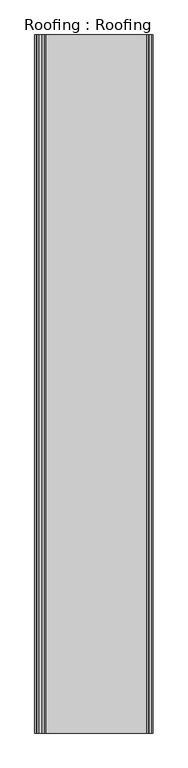
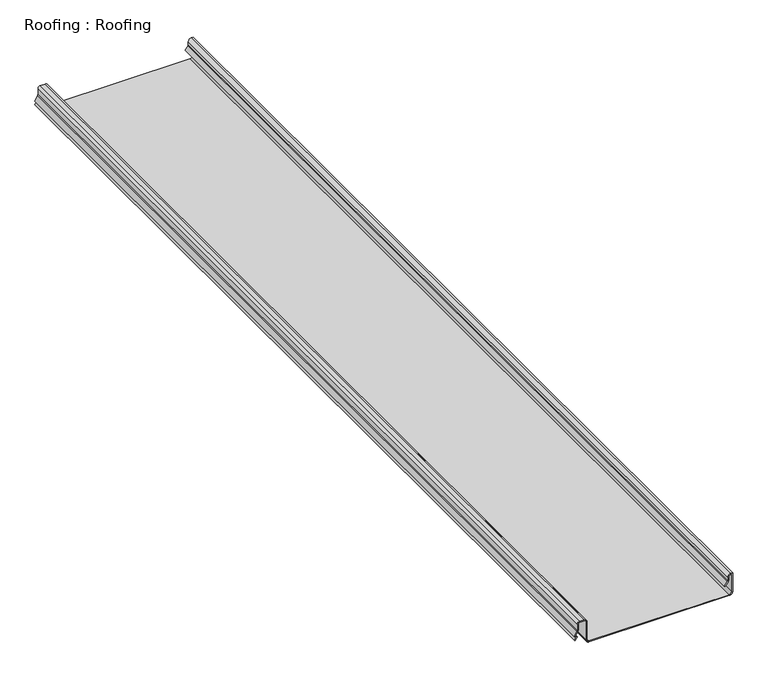
"""IFC4 building model written with IfcOpenShell, lengths in millimetres: proxy geometry, Roofing : Roofing."""

import ifcopenshell
import ifcopenshell.guid

model = None  # the IFC model being written
_history = None  # IfcOwnerHistory: only IFC2X3 demands one
_inside = {}  # id of a spatial element -> (the spatial element, [elements in it])
_under = {}  # id of a project, library or spatial element -> (it, [spatial elements below it])
_declared = {}  # id of a project -> (the project, [libraries it declares])
_typed = {}  # id of a type object -> (the type object, [elements of that type])
_made_of = {}  # id of a material, layer set ... -> (it, [elements and type objects made of it])


def new_model(schema):
    """Start an empty IFC model of exactly this schema.

    Asked for "IFC4X3", IfcOpenShell would pick the latest addendum, in which some entities
    have other attributes; the version numbers below select the first issue.
    IFC2X3 requires an IfcOwnerHistory on every rooted entity: one is made here for all.
    """
    global model, _history
    if schema == "IFC4X3":
        model = ifcopenshell.file(schema_version=(4, 3, 0, 0))
    else:
        model = ifcopenshell.file(schema=schema)
    _inside.clear()
    _under.clear()
    _declared.clear()
    _typed.clear()
    _made_of.clear()
    _history = None
    if model.schema == "IFC2X3":
        org = make("IfcOrganization", Name="unknown")
        user = make(
            "IfcPersonAndOrganization",
            ThePerson=make("IfcPerson", FamilyName="unknown"),
            TheOrganization=org,
        )
        app = make(
            "IfcApplication",
            ApplicationDeveloper=org,
            Version="unknown",
            ApplicationFullName="unknown",
            ApplicationIdentifier="unknown",
        )
        _history = make(
            "IfcOwnerHistory",
            OwningUser=user,
            OwningApplication=app,
            ChangeAction="ADDED",
            CreationDate=0,
        )
    return model


def make(cls, **values):
    """One entity of the class cls with the attributes given. An attribute that is None is left unset."""
    return model.create_entity(
        cls, **{name: value for name, value in values.items() if value is not None}
    )


def rooted(cls, **values):
    """An entity with a GlobalId (a new one), such as an element, a storey or a relation."""
    return make(cls, GlobalId=ifcopenshell.guid.new(), OwnerHistory=_history, **values)


def si_unit(unit_type, name, prefix=None):
    """IfcSIUnit, for example si_unit("LENGTHUNIT", "METRE", prefix="MILLI")."""
    return make("IfcSIUnit", UnitType=unit_type, Prefix=prefix, Name=name)


def assignment(units):
    """IfcUnitAssignment: the units of a project."""
    return None if units is None else make("IfcUnitAssignment", Units=units)


def point(xyz):
    """IfcCartesianPoint."""
    return None if xyz is None else make("IfcCartesianPoint", Coordinates=xyz)


def direction(xyz):
    """IfcDirection."""
    return None if xyz is None else make("IfcDirection", DirectionRatios=xyz)


def frame(location, z_axis=None, x_axis=None):
    """IfcAxis2Placement3D, a coordinate frame: its origin and axes. An axis left out is left unset."""
    return make(
        "IfcAxis2Placement3D",
        Location=point(location),
        Axis=direction(z_axis),
        RefDirection=direction(x_axis),
    )


def frame_2d(location, x_axis=None):
    """IfcAxis2Placement2D, a coordinate frame in the plane: its origin and x axis."""
    return make(
        "IfcAxis2Placement2D", Location=point(location), RefDirection=direction(x_axis)
    )


def origin():
    """The frame at (0, 0, 0) with its axes left unset."""
    return frame((0.0, 0.0, 0.0))


def place(relative_to, where):
    """IfcLocalPlacement: puts the frame where relative to a parent placement (None: the world)."""
    return make(
        "IfcLocalPlacement", PlacementRelTo=relative_to, RelativePlacement=where
    )


def context(
    kind, dimensions, precision=None, world=None, true_north=None, identifier=None
):
    """IfcGeometricRepresentationContext, for example the 3D "Model" context."""
    return make(
        "IfcGeometricRepresentationContext",
        ContextIdentifier=identifier,
        ContextType=kind,
        CoordinateSpaceDimension=dimensions,
        Precision=precision,
        WorldCoordinateSystem=world,
        TrueNorth=true_north,
    )


def project(units=None, contexts=None):
    """IfcProject with its units and contexts."""
    return rooted(
        "IfcProject",
        Name="project",
        RepresentationContexts=contexts,
        UnitsInContext=assignment(units),
    )


def spatial(cls, under=None, at=None, **own):
    """A site, building, storey or space (cls), placed at a placement, below another one or the project."""
    s = rooted(cls, ObjectPlacement=at, **own)
    if under is not None:
        _under.setdefault(under.id(), (under, []))[1].append(s)
    return s


def polyline(points):
    """IfcPolyline through the points."""
    return make("IfcPolyline", Points=[point(p) for p in points])


def circle_curve(where, radius):
    """IfcCircle in the frame where."""
    return make("IfcCircle", Position=where, Radius=radius)


def trimmed(basis, trim1, trim2, sense, master):
    """IfcTrimmedCurve: the piece of a basis curve between two trims."""
    return make(
        "IfcTrimmedCurve",
        BasisCurve=basis,
        Trim1=trim1,
        Trim2=trim2,
        SenseAgreement=sense,
        MasterRepresentation=master,
    )


def segment(curve, same_sense, transition):
    """IfcCompositeCurveSegment."""
    return make(
        "IfcCompositeCurveSegment",
        Transition=transition,
        SameSense=same_sense,
        ParentCurve=curve,
    )


def composite_curve(segments, self_intersect=None):
    """IfcCompositeCurve: segments joined end to end."""
    return make("IfcCompositeCurve", Segments=segments, SelfIntersect=self_intersect)


def outline(outer, holes=None, kind="AREA"):
    """IfcArbitraryClosedProfileDef: a profile drawn as a closed curve; with holes, ...WithVoids."""
    if holes is None:
        return make("IfcArbitraryClosedProfileDef", ProfileType=kind, OuterCurve=outer)
    return make(
        "IfcArbitraryProfileDefWithVoids",
        ProfileType=kind,
        OuterCurve=outer,
        InnerCurves=holes,
    )


def extrude(swept, where, along, depth):
    """IfcExtrudedAreaSolid: the profile swept, set in the frame where, extruded along a direction by depth."""
    return make(
        "IfcExtrudedAreaSolid",
        SweptArea=swept,
        Position=where,
        ExtrudedDirection=direction(along),
        Depth=depth,
    )


def shape(context_of_items, identifier, shape_type, items):
    """IfcShapeRepresentation: the items that make up one representation, for example the "Body"."""
    return make(
        "IfcShapeRepresentation",
        ContextOfItems=context_of_items,
        RepresentationIdentifier=identifier,
        RepresentationType=shape_type,
        Items=items,
    )


def source(mapping_origin, context_of_items, identifier, shape_type, items):
    """IfcRepresentationMap: a shape defined once, which mapped items show again and again."""
    return make(
        "IfcRepresentationMap",
        MappingOrigin=mapping_origin,
        MappedRepresentation=shape(context_of_items, identifier, shape_type, items),
    )


def transform(
    local_origin,
    x_axis=None,
    y_axis=None,
    z_axis=None,
    scale=None,
    scale2=None,
    scale3=None,
    uniform=True,
):
    """IfcCartesianTransformationOperator3D, or its non-uniform kind. x_axis, y_axis, z_axis: its Axis1, 2, 3."""
    if uniform:
        return make(
            "IfcCartesianTransformationOperator3D",
            Axis1=direction(x_axis),
            Axis2=direction(y_axis),
            LocalOrigin=point(local_origin),
            Scale=scale,
            Axis3=direction(z_axis),
        )
    return make(
        "IfcCartesianTransformationOperator3DnonUniform",
        Axis1=direction(x_axis),
        Axis2=direction(y_axis),
        LocalOrigin=point(local_origin),
        Scale=scale,
        Axis3=direction(z_axis),
        Scale2=scale2,
        Scale3=scale3,
    )


def mapped(mapping_source, mapping_target):
    """IfcMappedItem: shows the shape of a source again, moved by a transform."""
    return make(
        "IfcMappedItem", MappingSource=mapping_source, MappingTarget=mapping_target
    )


def made_of(thing, what):
    """Note that an element or type object is made of a material, layer set ...; save() writes the relation."""
    if what is not None:
        _made_of.setdefault(what.id(), (what, []))[1].append(thing)
    return thing


def element(
    cls,
    number,
    at=None,
    inside=None,
    cuts=None,
    type_object=None,
    material=None,
    context=None,
    identifier="Body",
    shape_type=None,
    held_by="IfcProductDefinitionShape",
    body=None,
    shapes=None,
    **own,
):
    """One element of the class cls, such as IfcWall. Its Tag is "e" and its number.

    at: its placement. inside: the storey or other place that contains it. cuts: it is an
    opening in that element (IfcRelVoidsElement). A single representation is given by context,
    identifier, shape_type and body (its items); several are given by shapes. held_by: the class
    of the entity that holds the representations. save() writes the other relations.
    """
    e = rooted(cls, Tag="e%d" % number, ObjectPlacement=at, **own)
    if body is not None:
        shapes = [shape(context, identifier, shape_type, body)]
    if shapes is not None:
        e.Representation = make(held_by, Representations=shapes)
    if inside is not None:
        _inside.setdefault(inside.id(), (inside, []))[1].append(e)
    if cuts is not None:
        rooted(
            "IfcRelVoidsElement", RelatingBuildingElement=cuts, RelatedOpeningElement=e
        )
    if type_object is not None:
        _typed.setdefault(type_object.id(), (type_object, []))[1].append(e)
    return made_of(e, material)


def aggregate(whole, parts):
    """IfcRelAggregates: a whole, such as a stair, and the parts it consists of."""
    return rooted("IfcRelAggregates", RelatingObject=whole, RelatedObjects=parts)


def save(model, path):
    """Write the relations noted so far, then the file.

    IfcRelAggregates (storeys below a building ...), IfcRelContainedInSpatialStructure (elements
    in a storey), IfcRelDefinesByType, IfcRelAssociatesMaterial and IfcRelDeclares: one each for
    every whole, place, type object, material and project.
    """
    for whole, parts in _under.values():
        aggregate(whole, parts)
    for where, things in _inside.values():
        rooted(
            "IfcRelContainedInSpatialStructure",
            RelatedElements=things,
            RelatingStructure=where,
        )
    for kind, things in _typed.values():
        rooted("IfcRelDefinesByType", RelatedObjects=things, RelatingType=kind)
    for what, things in _made_of.values():
        rooted("IfcRelAssociatesMaterial", RelatedObjects=things, RelatingMaterial=what)
    for by, libraries in _declared.values():
        rooted("IfcRelDeclares", RelatingContext=by, RelatedDefinitions=libraries)
    model.write(path)


def roofing_roofing_e53e7194(model_context):
    return source(origin(), model_context, "Body", "SweptSolid", [
        extrude(outline(composite_curve([segment(trimmed(circle_curve(frame_2d((43490.7540667, -5832.0326367)), 5.08), [point((43487.7710372, -5827.9207108))], [point((43490.7540667, -5826.9526367))], False, "CARTESIAN"), True, "CONTINUOUS"), segment(polyline([(43490.7540667, -5826.9526367), (43497.510625, -5826.9526367)]), True, "CONTINUOUS"), segment(trimmed(circle_curve(frame_2d((43497.510625, -5821.8726367)), 5.08), [point((43497.510625, -5826.9526367))], [point((43502.590625, -5821.8726367))], True, "CARTESIAN"), True, "CONTINUOUS"), segment(polyline([(43502.590625, -5821.8726367), (43502.590625, -5820.277832), (43462.8534375, -5820.277832)]), True, "CONTINUOUS"), segment(trimmed(circle_curve(frame_2d((43462.8534375, -5825.357832)), 5.08), [point((43462.8534375, -5820.277832))], [point((43457.7734375, -5825.357832))], True, "CARTESIAN"), True, "CONTINUOUS"), segment(polyline([(43457.7734375, -5825.357832), (43457.7734375, -6125.6319141)]), True, "CONTINUOUS"), segment(trimmed(circle_curve(frame_2d((43462.8534375, -6125.6319141)), 5.08), [point((43457.7734375, -6125.6319141))], [point((43462.8534375, -6130.7119141))], True, "CARTESIAN"), True, "CONTINUOUS"), segment(polyline([(43462.8534375, -6130.7119141), (43504.466875, -6130.7119141)]), True, "CONTINUOUS"), segment(trimmed(circle_curve(frame_2d((43504.466875, -6135.7919141)), 5.08), [point((43504.466875, -6130.7119141))], [point((43509.546875, -6135.7919141))], False, "CARTESIAN"), True, "CONTINUOUS"), segment(polyline([(43509.546875, -6135.7919141), (43509.546875, -6145.799691)]), True, "CONTINUOUS"), segment(trimmed(circle_curve(frame_2d((43504.466875, -6145.799691)), 5.08), [point((43509.546875, -6145.799691))], [point((43504.466875, -6150.879691))], False, "CARTESIAN"), True, "CONTINUOUS"), segment(polyline([(43504.466875, -6150.879691), (43491.2843008, -6150.879691)]), True, "CONTINUOUS"), segment(trimmed(circle_curve(frame_2d((43491.2843008, -6155.959691)), 5.08), [point((43491.2843008, -6150.879691))], [point((43488.7802894, -6151.5396993))], True, "CARTESIAN"), True, "CONTINUOUS"), segment(polyline([(43488.7802894, -6151.5396993), (43478.2226563, -6157.5208042), (43475.78125, -6153.3567417), (43470.1796875, -6157.3557652), (43469.0176138, -6155.7280107), (43476.399929, -6150.4576863), (43478.9513272, -6154.8093511), (43487.7944581, -6149.7995451)]), True, "CONTINUOUS"), segment(trimmed(circle_curve(frame_2d((43491.2843008, -6155.959691)), 7.08), [point((43487.7944581, -6149.7995451))], [point((43491.2843008, -6148.879691))], False, "CARTESIAN"), True, "CONTINUOUS"), segment(polyline([(43491.2843008, -6148.879691), (43504.466875, -6148.879691)]), True, "CONTINUOUS"), segment(trimmed(circle_curve(frame_2d((43504.466875, -6145.799691)), 3.08), [point((43504.466875, -6148.879691))], [point((43507.546875, -6145.799691))], True, "CARTESIAN"), True, "CONTINUOUS"), segment(polyline([(43507.546875, -6145.799691), (43507.546875, -6135.7919141)]), True, "CONTINUOUS"), segment(trimmed(circle_curve(frame_2d((43504.466875, -6135.7919141)), 3.08), [point((43507.546875, -6135.7919141))], [point((43504.466875, -6132.7119141))], True, "CARTESIAN"), True, "CONTINUOUS"), segment(polyline([(43504.466875, -6132.7119141), (43462.8534375, -6132.7119141)]), True, "CONTINUOUS"), segment(trimmed(circle_curve(frame_2d((43462.8534375, -6125.6319141)), 7.08), [point((43462.8534375, -6132.7119141))], [point((43455.7734375, -6125.6319141))], False, "CARTESIAN"), True, "CONTINUOUS"), segment(polyline([(43455.7734375, -6125.6319141), (43455.7734375, -5825.357832)]), True, "CONTINUOUS"), segment(trimmed(circle_curve(frame_2d((43462.8534375, -5825.357832)), 7.08), [point((43455.7734375, -5825.357832))], [point((43462.8534375, -5818.277832))], False, "CARTESIAN"), True, "CONTINUOUS"), segment(polyline([(43462.8534375, -5818.277832), (43504.590625, -5818.277832), (43504.590625, -5821.8726367)]), True, "CONTINUOUS"), segment(trimmed(circle_curve(frame_2d((43497.510625, -5821.8726367)), 7.08), [point((43504.590625, -5821.8726367))], [point((43497.510625, -5828.9526367))], False, "CARTESIAN"), True, "CONTINUOUS"), segment(polyline([(43497.510625, -5828.9526367), (43490.7540667, -5828.9526367)]), True, "CONTINUOUS"), segment(trimmed(circle_curve(frame_2d((43490.7540667, -5832.0326367)), 3.08), [point((43490.7540667, -5828.9526367))], [point((43488.9454582, -5829.5395793))], True, "CARTESIAN"), True, "CONTINUOUS"), segment(polyline([(43488.9454582, -5829.5395793), (43480.4712961, -5835.6872279), (43479.296875, -5834.0683594), (43487.7710372, -5827.9207108)]), True, "CONTINUOUS")], self_intersect=False)), frame((0.0, 7982.1531721, 0.0), z_axis=(0.0, 1.0, 0.0), x_axis=(0.0, 0.0, 1.0)), (0.0, 0.0, 1.0), 2000.0),
    ])


if __name__ == "__main__":
    model = new_model("IFC4")
    model_context = context("Model", 3, world=origin())
    ifc_project = project(units=[si_unit("LENGTHUNIT", "METRE", prefix="MILLI")], contexts=[model_context])
    site = spatial("IfcSite", under=ifc_project)
    building = spatial("IfcBuilding", under=site)
    placement = place(None, origin())
    roofing_roofing_shape = roofing_roofing_e53e7194(model_context)
    element("IfcBuildingElementProxy", 1, Name="Roofing : Roofing", ObjectType="Roofing : Roofing", at=placement, inside=building, context=model_context, shape_type="MappedRepresentation", body=[
        mapped(roofing_roofing_shape, transform((0.0, 0.0, 0.0), x_axis=(1.0, 0.0, 0.0), y_axis=(0.0, 1.0, 0.0), z_axis=(0.0, 0.0, 1.0))),
    ])
    save(model, "model.ifc")

# Revit data of these elements
# Type "Roofing : Roofing"
#   NameOverride = "Roofing"
# Element 1 (IfcBuildingElementProxy, "Roofing : Roofing")
#   Materials on its faces: "STANDING SEAM METAL ROOF"
# Materials
#   "STANDING SEAM METAL ROOF": class "Unassigned", colour RGB 128 128 128, transparency 0
